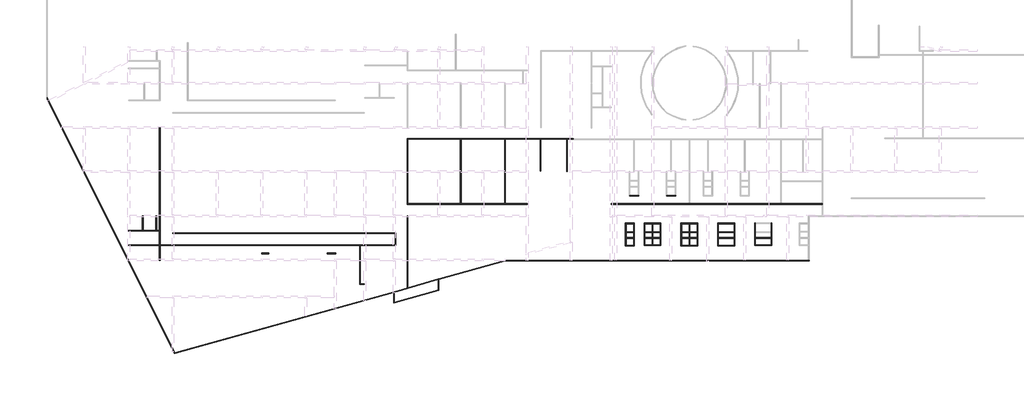
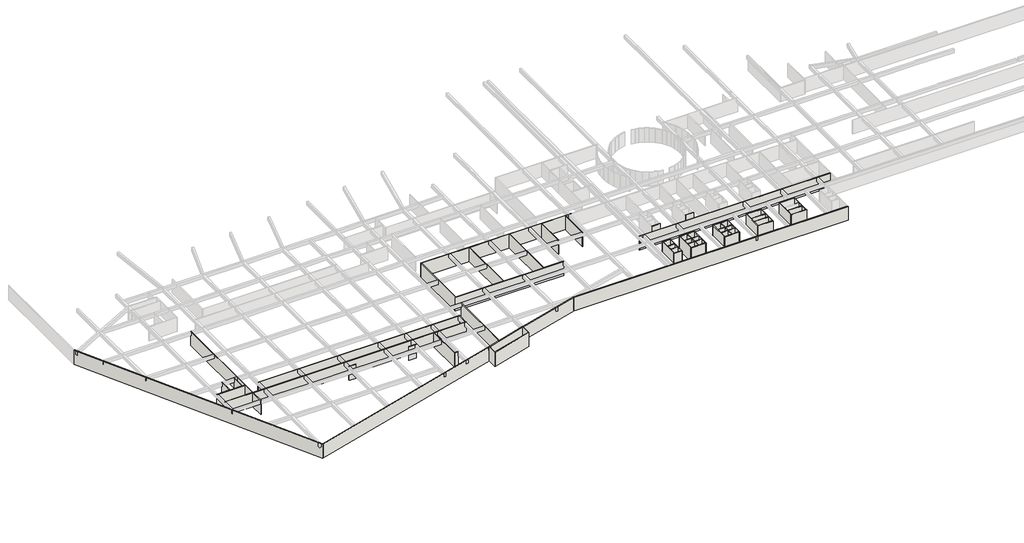
# One storey, part 1 of 8: 60 walls.
# Revit data of these elements (continued)
# Area, not placed, upper offset 0 mm, lower offset 0 mm
#   Number = "194"
#   Name = "fire_compart"
# Area, not placed, upper offset 0 mm, lower offset 0 mm
#   Number = "195"
#   Name = "面积"
# Area, not placed, upper offset 0 mm, lower offset 0 mm
#   Number = "196"
#   Name = "fire_compart"
# Area, not placed, upper offset 0 mm, lower offset 0 mm
#   Number = "197"
#   Name = "fire_compart"
# Area, not placed, upper offset 0 mm, lower offset 0 mm
#   Number = "198"
#   Name = "fire_compart"
# Area, not placed, upper offset 0 mm, lower offset 0 mm
#   Number = "199"
#   Name = "fire_compart"
# Area, not placed, upper offset 0 mm, lower offset 0 mm
#   Number = "200"
#   Name = "fire_compart"
# Area, not placed, upper offset 0 mm, lower offset 0 mm
#   Number = "201"
#   Name = "fire_compart"
# Area, not placed, upper offset 0 mm, lower offset 0 mm
#   Number = "202"
#   Name = "fire_compart"
# Area, not placed, upper offset 0 mm, lower offset 0 mm
#   Number = "203"
#   Name = "fire_compart"
# Area, not placed, upper offset 0 mm, lower offset 0 mm
#   Number = "105"
#   Name = "main_building"
# Room, not placed, phase "新构造", upper offset 0 mm, lower offset 0 mm
#   Number = "11"
#   Name = "房间"
# Area, not placed, upper offset 0 mm, lower offset 0 mm
#   Number = "106"
#   Name = "main_building"
# Room, not placed, phase "新构造", upper offset 0 mm, lower offset 0 mm
#   Number = "12"
#   Name = "房间"
# Room, not placed, phase "新构造", upper offset 0 mm, lower offset 0 mm
#   Number = "13"
#   Name = "房间"
# Room, not placed, phase "新构造", upper offset 0 mm, lower offset 0 mm
#   Number = "14"
#   Name = "房间"
# Room, not placed, phase "新构造", upper offset 0 mm, lower offset 0 mm
#   Number = "15"
#   Name = "房间"
# Room, not placed, phase "新构造", upper offset 0 mm, lower offset 0 mm
#   Number = "16"
#   Name = "房间"
# Room, not placed, phase "新构造", upper offset 0 mm, lower offset 0 mm
#   Number = "17"
#   Name = "房间"
# Area, not placed, upper offset 0 mm, lower offset 0 mm
#   Number = "204"
#   Name = "main_building"
# Area, not placed, upper offset 0 mm, lower offset 0 mm
#   Number = "41"
#   Name = "main_building"
# Area, not placed, upper offset 0 mm, lower offset 0 mm
#   Number = "42"
#   Name = "main_building"
# Area, not placed, upper offset 0 mm, lower offset 0 mm
#   Number = "43"
#   Name = "main_building"
# Area, not placed, upper offset 0 mm, lower offset 0 mm
#   Number = "44"
#   Name = "main_building"
# Area, not placed, upper offset 0 mm, lower offset 0 mm
#   Number = "45"
#   Name = "main_building"
# Area, not placed, upper offset 0 mm, lower offset 0 mm
#   Number = "46"
#   Name = "main_building"
# Area, not placed, upper offset 0 mm, lower offset 0 mm
#   Number = "47"
#   Name = "main_building"
# Area, not placed, upper offset 0 mm, lower offset 0 mm
#   Number = "48"
#   Name = "main_building"
# Area, not placed, upper offset 0 mm, lower offset 0 mm
#   Number = "49"
#   Name = "main_building"
# Area, not placed, upper offset 0 mm, lower offset 0 mm
#   Number = "50"
#   Name = "main_building"
# Area, not placed, upper offset 0 mm, lower offset 0 mm
#   Number = "51"
#   Name = "fire_compart"
# Area, not placed, upper offset 0 mm, lower offset 0 mm
#   Number = "205"
#   Name = "main_building"
# Area, not placed, upper offset 0 mm, lower offset 0 mm
#   Number = "107"
#   Name = "main_building"
# Area, not placed, upper offset 0 mm, lower offset 0 mm
#   Number = "52"
#   Name = "fire_compart"
# Area, not placed, upper offset 0 mm, lower offset 0 mm
#   Number = "53"
#   Name = "fire_compart"
# Area, not placed, upper offset 0 mm, lower offset 0 mm
#   Number = "54"
#   Name = "fire_compart"
# Area, not placed, upper offset 0 mm, lower offset 0 mm
#   Number = "206"
#   Name = "main_building"
# Area, not placed, upper offset 0 mm, lower offset 0 mm
#   Number = "148"
#   Name = "main_building"
# Area, not placed, upper offset 0 mm, lower offset 0 mm
#   Number = "55"
#   Name = "fire_compart"
# Area, not placed, upper offset 0 mm, lower offset 0 mm
#   Number = "56"
#   Name = "fire_compart"
# Area, not placed, upper offset 0 mm, lower offset 0 mm
#   Number = "207"
#   Name = "main_building"
# Area, not placed, upper offset 0 mm, lower offset 0 mm
#   Number = "57"
#   Name = "fire_compart"
# Area, not placed, upper offset 0 mm, lower offset 0 mm
#   Number = "24"
#   Name = "fire_compart"
# Area, not placed, upper offset 0 mm, lower offset 0 mm
#   Number = "58"
#   Name = "fire_compart"
# Area, not placed, upper offset 0 mm, lower offset 0 mm
#   Number = "208"
#   Name = "main_building"
# Area, not placed, upper offset 0 mm, lower offset 0 mm
#   Number = "209"
#   Name = "面积"
# Area, not placed, upper offset 0 mm, lower offset 0 mm
#   Number = "59"
#   Name = "fire_compart"
# Area, not placed, upper offset 0 mm, lower offset 0 mm
#   Number = "149"
#   Name = "main_building"
# Room, not placed, phase "新构造", upper offset 0 mm, lower offset 0 mm
#   Number = "1"
#   Name = "客餐厅"
# Room, not placed, phase "新构造", upper offset 0 mm, lower offset 0 mm
#   Number = "2"
#   Name = "阳台"
# Area, not placed, upper offset 0 mm, lower offset 0 mm
#   Number = "210"
#   Name = "main_building"
# Room, not placed, phase "新构造", upper offset 0 mm, lower offset 0 mm
#   Number = "3"
#   Name = "次卧"
# Room, not placed, phase "新构造", upper offset 0 mm, lower offset 0 mm
#   Number = "4"
#   Name = "厨房"
# Area, not placed, upper offset 0 mm, lower offset 0 mm
#   Number = "108"
#   Name = "main_building"
# Room, not placed, phase "新构造", upper offset 0 mm, lower offset 0 mm
#   Number = "5"
#   Name = "卫生间"
# Room, not placed, phase "新构造", upper offset 0 mm, lower offset 0 mm
#   Number = "6"
#   Name = "次卧"
# Room, not placed, phase "新构造", upper offset 0 mm, lower offset 0 mm
#   Number = "7"
#   Name = "主卧"
# Area, not placed, upper offset 0 mm, lower offset 0 mm
#   Number = "60"
#   Name = "fire_compart"
# Area, not placed, upper offset 0 mm, lower offset 0 mm
#   Number = "61"
#   Name = "fire_compart"
# Area, not placed, upper offset 0 mm, lower offset 0 mm
#   Number = "62"
#   Name = "fire_compart"
# Area, not placed, upper offset 0 mm, lower offset 0 mm
#   Number = "63"
#   Name = "fire_compart"
# Area, not placed, upper offset 0 mm, lower offset 0 mm
#   Number = "83"
#   Name = "fire_compart"
# Area, not placed, upper offset 0 mm, lower offset 0 mm
#   Number = "84"
#   Name = "main_building"
# Area, not placed, upper offset 0 mm, lower offset 0 mm
#   Number = "150"
#   Name = "main_building"
# Area, not placed, upper offset 0 mm, lower offset 0 mm
#   Number = "151"
#   Name = "main_building"
# Area, not placed, upper offset 0 mm, lower offset 0 mm
#   Number = "109"
#   Name = "main_building"
# Area, not placed, upper offset 0 mm, lower offset 0 mm
#   Number = "152"
#   Name = "main_building"
# Area, not placed, upper offset 0 mm, lower offset 0 mm
#   Number = "1"
#   Name = "面积"
# Area, not placed, upper offset 0 mm, lower offset 0 mm
#   Number = "2"
#   Name = "防火区域1"
# Area, not placed, upper offset 0 mm, lower offset 0 mm
#   Number = "25"
#   Name = "fire_compart"
# Area, not placed, upper offset 0 mm, lower offset 0 mm
#   Number = "26"
#   Name = "fire_compart"
# Area, not placed, upper offset 0 mm, lower offset 0 mm
#   Number = "27"
#   Name = "fire_compart"
# Area, not placed, upper offset 0 mm, lower offset 0 mm
#   Number = "153"
#   Name = "main_building"
# Area, not placed, upper offset 0 mm, lower offset 0 mm
#   Number = "85"
#   Name = "fire_compart"
# Area, not placed, upper offset 0 mm, lower offset 0 mm
#   Number = "86"
#   Name = "main_building"
# Area, not placed, upper offset 0 mm, lower offset 0 mm
#   Number = "87"
#   Name = "main_building"
# Area, not placed, upper offset 0 mm, lower offset 0 mm
#   Number = "154"
#   Name = "main_building"
# Area, not placed, upper offset 0 mm, lower offset 0 mm
#   Number = "3"
#   Name = "fire_compart_1"
# Area, not placed, upper offset 0 mm, lower offset 0 mm
#   Number = "155"
#   Name = "main_building"
# Area, not placed, upper offset 0 mm, lower offset 0 mm
#   Number = "110"
#   Name = "main_building"
# Area, not placed, upper offset 0 mm, lower offset 0 mm
#   Number = "88"
#   Name = "fire_compart"
# Area, not placed, upper offset 0 mm, lower offset 0 mm
#   Number = "28"
#   Name = "面积"
# Area, not placed, upper offset 0 mm, lower offset 0 mm
#   Number = "211"
#   Name = "fire_compart"
# Area, not placed, upper offset 0 mm, lower offset 0 mm
#   Number = "29"
#   Name = "main_building"
# Area, not placed, upper offset 0 mm, lower offset 0 mm
#   Number = "30"
#   Name = "main_building"
# Area, not placed, upper offset 0 mm, lower offset 0 mm
#   Number = "212"
#   Name = "fire_compart"
# Area, not placed, upper offset 0 mm, lower offset 0 mm
#   Number = "89"
#   Name = "main_building"
# Area, not placed, upper offset 0 mm, lower offset 0 mm
#   Number = "111"
#   Name = "main_building"
# Area, not placed, upper offset 0 mm, lower offset 0 mm
#   Number = "90"
#   Name = "fire_compart"
# Area, not placed, upper offset 0 mm, lower offset 0 mm
#   Number = "213"
#   Name = "fire_compart"
# Area, not placed, upper offset 0 mm, lower offset 0 mm
#   Number = "214"
#   Name = "fire_compart"
# Area, not placed, upper offset 0 mm, lower offset 0 mm
#   Number = "4"
#   Name = "fire_compart_2"
# Area, not placed, upper offset 0 mm, lower offset 0 mm
#   Number = "215"
#   Name = "fire_compart"
# Area, not placed, upper offset 0 mm, lower offset 0 mm
#   Number = "91"
#   Name = "main_building"
# Area, not placed, upper offset 0 mm, lower offset 0 mm
#   Number = "31"
#   Name = "main_building"
# Area, not placed, upper offset 0 mm, lower offset 0 mm
#   Number = "32"
#   Name = "main_building"
# Area, not placed, upper offset 0 mm, lower offset 0 mm
#   Number = "33"
#   Name = "main_building"
# Area, not placed, upper offset 0 mm, lower offset 0 mm
#   Number = "34"
#   Name = "main_building"
# Area, not placed, upper offset 0 mm, lower offset 0 mm
#   Number = "35"
#   Name = "main_building"
# Area, not placed, upper offset 0 mm, lower offset 0 mm
#   Number = "5"
#   Name = "fire_compart_3"
# Area, not placed, upper offset 0 mm, lower offset 0 mm
#   Number = "156"
#   Name = "fire_compart"
# Area, not placed, upper offset 0 mm, lower offset 0 mm
#   Number = "157"
#   Name = "fire_compart"
# Area, not placed, upper offset 0 mm, lower offset 0 mm
#   Number = "158"
#   Name = "fire_compart"
# Area, not placed, upper offset 0 mm, lower offset 0 mm
#   Number = "160"
#   Name = "fire_compart"
# Area, not placed, upper offset 0 mm, lower offset 0 mm
#   Number = "92"
#   Name = "fire_compart"
# Area, not placed, upper offset 0 mm, lower offset 0 mm
#   Number = "93"
#   Name = "main_building"
# Area, not placed, upper offset 0 mm, lower offset 0 mm
#   Number = "94"
#   Name = "main_building"
# Area, not placed, upper offset 0 mm, lower offset 0 mm
#   Number = "95"
#   Name = "fire_compart"
# Area, not placed, upper offset 0 mm, lower offset 0 mm
#   Number = "96"
#   Name = "main_building"
# Area, not placed, upper offset 0 mm, lower offset 0 mm
#   Number = "97"
#   Name = "main_building"
# Area, not placed, upper offset 0 mm, lower offset 0 mm
#   Number = "6"
#   Name = "fire_compart_4"
# Area, not placed, upper offset 0 mm, lower offset 0 mm
#   Number = "98"
#   Name = "fire_compart"
# Area, not placed, upper offset 0 mm, lower offset 0 mm
#   Number = "99"
#   Name = "main_building"
# Area, not placed, upper offset 0 mm, lower offset 0 mm
#   Number = "161"
#   Name = "main_building"
# Area, not placed, upper offset 0 mm, lower offset 0 mm
#   Number = "7"
#   Name = "fire_compart_5"
# Area, not placed, upper offset 0 mm, lower offset 0 mm
#   Number = "162"
#   Name = "main_building"
# Area, not placed, upper offset 0 mm, lower offset 0 mm
#   Number = "112"
#   Name = "main_building"
# Area, not placed, upper offset 0 mm, lower offset 0 mm
#   Number = "113"
#   Name = "main_building"
# Area, not placed, upper offset 0 mm, lower offset 0 mm
#   Number = "177"
#   Name = "main_building"
# Area at (338056.897, 32393.027) mm, upper offset 0 mm, lower offset 0 mm
#   Number = "216"
#   Name = "main_building"
# Room, not placed, phase "新构造", upper offset 0 mm, lower offset 0 mm
#   Number = "8"
#   Name = "客餐厅"
# Area at (376762.564, 36199.141) mm, upper offset 0 mm, lower offset 0 mm
#   Number = "217"
#   Name = "main_building"
# Area, not placed, upper offset 0 mm, lower offset 0 mm
#   Number = "114"
#   Name = "main_building"
# Area at (476149.092, 25478.212) mm, upper offset 0 mm, lower offset 0 mm
#   Number = "218"
#   Name = "main_building"
# Area, not placed, upper offset 0 mm, lower offset 0 mm
#   Number = "8"
#   Name = "fire_compart_6"
# Area, not placed, upper offset 0 mm, lower offset 0 mm
#   Number = "178"
#   Name = "main_building"
# Area, not placed, upper offset 0 mm, lower offset 0 mm
#   Number = "163"
#   Name = "main_building"
# Area, not placed, upper offset 0 mm, lower offset 0 mm
#   Number = "115"
#   Name = "main_building"
# Area, not placed, upper offset 0 mm, lower offset 0 mm
#   Number = "179"
#   Name = "main_building"
# Area, not placed, upper offset 0 mm, lower offset 0 mm
#   Number = "164"
#   Name = "main_building"
# Area, not placed, upper offset 0 mm, lower offset 0 mm
#   Number = "116"
#   Name = "main_building"
# Area, not placed, upper offset 0 mm, lower offset 0 mm
#   Number = "180"
#   Name = "main_building"
# Area, not placed, upper offset 0 mm, lower offset 0 mm
#   Number = "117"
#   Name = "main_building"
# Area, not placed, upper offset 0 mm, lower offset 0 mm
#   Number = "181"
#   Name = "main_building"
